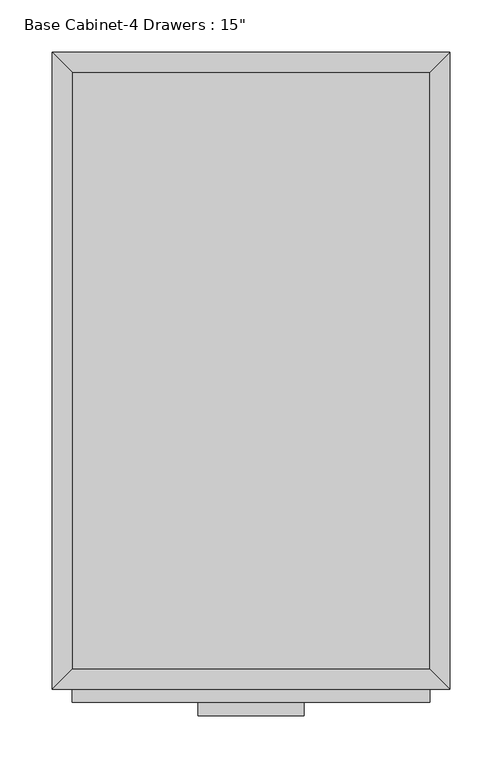
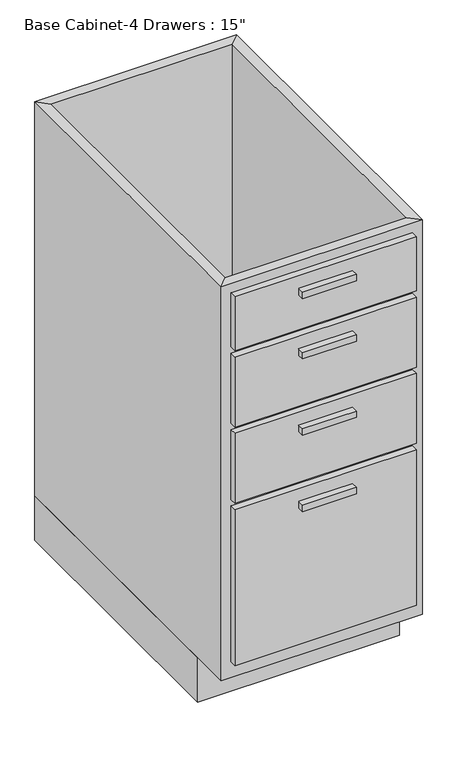
"""IFC4 building model written with IfcOpenShell, lengths in millimetres: furniture geometry."""

import ifcopenshell
import ifcopenshell.guid

model = None  # the IFC model being written
_history = None  # IfcOwnerHistory: only IFC2X3 demands one
_inside = {}  # id of a spatial element -> (the spatial element, [elements in it])
_under = {}  # id of a project, library or spatial element -> (it, [spatial elements below it])
_declared = {}  # id of a project -> (the project, [libraries it declares])
_typed = {}  # id of a type object -> (the type object, [elements of that type])
_made_of = {}  # id of a material, layer set ... -> (it, [elements and type objects made of it])


def new_model(schema):
    """Start an empty IFC model of exactly this schema.

    Asked for "IFC4X3", IfcOpenShell would pick the latest addendum, in which some entities
    have other attributes; the version numbers below select the first issue.
    IFC2X3 requires an IfcOwnerHistory on every rooted entity: one is made here for all.
    """
    global model, _history
    if schema == "IFC4X3":
        model = ifcopenshell.file(schema_version=(4, 3, 0, 0))
    else:
        model = ifcopenshell.file(schema=schema)
    _inside.clear()
    _under.clear()
    _declared.clear()
    _typed.clear()
    _made_of.clear()
    _history = None
    if model.schema == "IFC2X3":
        org = make("IfcOrganization", Name="unknown")
        user = make(
            "IfcPersonAndOrganization",
            ThePerson=make("IfcPerson", FamilyName="unknown"),
            TheOrganization=org,
        )
        app = make(
            "IfcApplication",
            ApplicationDeveloper=org,
            Version="unknown",
            ApplicationFullName="unknown",
            ApplicationIdentifier="unknown",
        )
        _history = make(
            "IfcOwnerHistory",
            OwningUser=user,
            OwningApplication=app,
            ChangeAction="ADDED",
            CreationDate=0,
        )
    return model


def make(cls, **values):
    """One entity of the class cls with the attributes given. An attribute that is None is left unset."""
    return model.create_entity(
        cls, **{name: value for name, value in values.items() if value is not None}
    )


def rooted(cls, **values):
    """An entity with a GlobalId (a new one), such as an element, a storey or a relation."""
    return make(cls, GlobalId=ifcopenshell.guid.new(), OwnerHistory=_history, **values)


def si_unit(unit_type, name, prefix=None):
    """IfcSIUnit, for example si_unit("LENGTHUNIT", "METRE", prefix="MILLI")."""
    return make("IfcSIUnit", UnitType=unit_type, Prefix=prefix, Name=name)


def assignment(units):
    """IfcUnitAssignment: the units of a project."""
    return None if units is None else make("IfcUnitAssignment", Units=units)


def point(xyz):
    """IfcCartesianPoint."""
    return None if xyz is None else make("IfcCartesianPoint", Coordinates=xyz)


def direction(xyz):
    """IfcDirection."""
    return None if xyz is None else make("IfcDirection", DirectionRatios=xyz)


def frame(location, z_axis=None, x_axis=None):
    """IfcAxis2Placement3D, a coordinate frame: its origin and axes. An axis left out is left unset."""
    return make(
        "IfcAxis2Placement3D",
        Location=point(location),
        Axis=direction(z_axis),
        RefDirection=direction(x_axis),
    )


def origin():
    """The frame at (0, 0, 0) with its axes left unset."""
    return frame((0.0, 0.0, 0.0))


def origin_with_axes():
    """The frame at (0, 0, 0) with the z axis (0, 0, 1) and the x axis (1, 0, 0) written out."""
    return frame((0.0, 0.0, 0.0), z_axis=(0.0, 0.0, 1.0), x_axis=(1.0, 0.0, 0.0))


def place(relative_to, where):
    """IfcLocalPlacement: puts the frame where relative to a parent placement (None: the world)."""
    return make(
        "IfcLocalPlacement", PlacementRelTo=relative_to, RelativePlacement=where
    )


def context(
    kind, dimensions, precision=None, world=None, true_north=None, identifier=None
):
    """IfcGeometricRepresentationContext, for example the 3D "Model" context."""
    return make(
        "IfcGeometricRepresentationContext",
        ContextIdentifier=identifier,
        ContextType=kind,
        CoordinateSpaceDimension=dimensions,
        Precision=precision,
        WorldCoordinateSystem=world,
        TrueNorth=true_north,
    )


def project(units=None, contexts=None):
    """IfcProject with its units and contexts."""
    return rooted(
        "IfcProject",
        Name="project",
        RepresentationContexts=contexts,
        UnitsInContext=assignment(units),
    )


def spatial(cls, under=None, at=None, **own):
    """A site, building, storey or space (cls), placed at a placement, below another one or the project."""
    s = rooted(cls, ObjectPlacement=at, **own)
    if under is not None:
        _under.setdefault(under.id(), (under, []))[1].append(s)
    return s


def polyline(points):
    """IfcPolyline through the points."""
    return make("IfcPolyline", Points=[point(p) for p in points])


def outline(outer, holes=None, kind="AREA"):
    """IfcArbitraryClosedProfileDef: a profile drawn as a closed curve; with holes, ...WithVoids."""
    if holes is None:
        return make("IfcArbitraryClosedProfileDef", ProfileType=kind, OuterCurve=outer)
    return make(
        "IfcArbitraryProfileDefWithVoids",
        ProfileType=kind,
        OuterCurve=outer,
        InnerCurves=holes,
    )


def extrude(swept, where, along, depth):
    """IfcExtrudedAreaSolid: the profile swept, set in the frame where, extruded along a direction by depth."""
    return make(
        "IfcExtrudedAreaSolid",
        SweptArea=swept,
        Position=where,
        ExtrudedDirection=direction(along),
        Depth=depth,
    )


def faces_of(points, faces, orient=None, outer=None):
    """IfcFace entities. A face is a list of loops; a loop is a list of indices into points, from 0.

    orient and outer hold one flag for each loop. By default every Orientation is true, the
    first loop of a face is its IfcFaceOuterBound and the others are IfcFaceBound.
    """
    made = []
    for i, loops in enumerate(faces):
        bounds = []
        for j, loop in enumerate(loops):
            is_outer = j == 0 if outer is None else outer[i][j]
            bounds.append(
                make(
                    "IfcFaceOuterBound" if is_outer else "IfcFaceBound",
                    Bound=make("IfcPolyLoop", Polygon=[points[k] for k in loop]),
                    Orientation=True if orient is None else orient[i][j],
                )
            )
        made.append(make("IfcFace", Bounds=bounds))
    return made


def faceted_brep(points, faces, orient=None, outer=None, voids=None):
    """IfcFacetedBrep: a solid bounded by flat faces; with voids (closed shells), ...WithVoids."""
    shared = [point(p) for p in points]
    hull = make("IfcClosedShell", CfsFaces=faces_of(shared, faces, orient, outer))
    if voids is None:
        return make("IfcFacetedBrep", Outer=hull)
    return make(
        "IfcFacetedBrepWithVoids",
        Outer=hull,
        Voids=[
            make(cls, CfsFaces=faces_of(shared, fs, o, b)) for cls, fs, o, b in voids
        ],
    )


def shape(context_of_items, identifier, shape_type, items):
    """IfcShapeRepresentation: the items that make up one representation, for example the "Body"."""
    return make(
        "IfcShapeRepresentation",
        ContextOfItems=context_of_items,
        RepresentationIdentifier=identifier,
        RepresentationType=shape_type,
        Items=items,
    )


def source(mapping_origin, context_of_items, identifier, shape_type, items):
    """IfcRepresentationMap: a shape defined once, which mapped items show again and again."""
    return make(
        "IfcRepresentationMap",
        MappingOrigin=mapping_origin,
        MappedRepresentation=shape(context_of_items, identifier, shape_type, items),
    )


def transform(
    local_origin,
    x_axis=None,
    y_axis=None,
    z_axis=None,
    scale=None,
    scale2=None,
    scale3=None,
    uniform=True,
):
    """IfcCartesianTransformationOperator3D, or its non-uniform kind. x_axis, y_axis, z_axis: its Axis1, 2, 3."""
    if uniform:
        return make(
            "IfcCartesianTransformationOperator3D",
            Axis1=direction(x_axis),
            Axis2=direction(y_axis),
            LocalOrigin=point(local_origin),
            Scale=scale,
            Axis3=direction(z_axis),
        )
    return make(
        "IfcCartesianTransformationOperator3DnonUniform",
        Axis1=direction(x_axis),
        Axis2=direction(y_axis),
        LocalOrigin=point(local_origin),
        Scale=scale,
        Axis3=direction(z_axis),
        Scale2=scale2,
        Scale3=scale3,
    )


def mapped(mapping_source, mapping_target):
    """IfcMappedItem: shows the shape of a source again, moved by a transform."""
    return make(
        "IfcMappedItem", MappingSource=mapping_source, MappingTarget=mapping_target
    )


def made_of(thing, what):
    """Note that an element or type object is made of a material, layer set ...; save() writes the relation."""
    if what is not None:
        _made_of.setdefault(what.id(), (what, []))[1].append(thing)
    return thing


def element(
    cls,
    number,
    at=None,
    inside=None,
    cuts=None,
    type_object=None,
    material=None,
    context=None,
    identifier="Body",
    shape_type=None,
    held_by="IfcProductDefinitionShape",
    body=None,
    shapes=None,
    **own,
):
    """One element of the class cls, such as IfcWall. Its Tag is "e" and its number.

    at: its placement. inside: the storey or other place that contains it. cuts: it is an
    opening in that element (IfcRelVoidsElement). A single representation is given by context,
    identifier, shape_type and body (its items); several are given by shapes. held_by: the class
    of the entity that holds the representations. save() writes the other relations.
    """
    e = rooted(cls, Tag="e%d" % number, ObjectPlacement=at, **own)
    if body is not None:
        shapes = [shape(context, identifier, shape_type, body)]
    if shapes is not None:
        e.Representation = make(held_by, Representations=shapes)
    if inside is not None:
        _inside.setdefault(inside.id(), (inside, []))[1].append(e)
    if cuts is not None:
        rooted(
            "IfcRelVoidsElement", RelatingBuildingElement=cuts, RelatedOpeningElement=e
        )
    if type_object is not None:
        _typed.setdefault(type_object.id(), (type_object, []))[1].append(e)
    return made_of(e, material)


def aggregate(whole, parts):
    """IfcRelAggregates: a whole, such as a stair, and the parts it consists of."""
    return rooted("IfcRelAggregates", RelatingObject=whole, RelatedObjects=parts)


def save(model, path):
    """Write the relations noted so far, then the file.

    IfcRelAggregates (storeys below a building ...), IfcRelContainedInSpatialStructure (elements
    in a storey), IfcRelDefinesByType, IfcRelAssociatesMaterial and IfcRelDeclares: one each for
    every whole, place, type object, material and project.
    """
    for whole, parts in _under.values():
        aggregate(whole, parts)
    for where, things in _inside.values():
        rooted(
            "IfcRelContainedInSpatialStructure",
            RelatedElements=things,
            RelatingStructure=where,
        )
    for kind, things in _typed.values():
        rooted("IfcRelDefinesByType", RelatedObjects=things, RelatingType=kind)
    for what, things in _made_of.values():
        rooted("IfcRelAssociatesMaterial", RelatedObjects=things, RelatingMaterial=what)
    for by, libraries in _declared.values():
        rooted("IfcRelDeclares", RelatingContext=by, RelatedDefinitions=libraries)
    model.write(path)


def furniture_a33faecb(model_context):
    return source(origin(), model_context, "Body", "SolidModel", [
        extrude(outline(polyline([(69.5377049, -635.0), (-32.0622951, -635.0), (-32.0622951, -622.3), (69.5377049, -622.3), (69.5377049, -635.0)])), frame((0.0, 0.0, 819.15), z_axis=(0.0, 0.0, 1.0), x_axis=(1.0, 0.0, 0.0)), (0.0, 0.0, 1.0), 12.7),
        extrude(outline(polyline([(69.5377049, -635.0), (-32.0622951, -635.0), (-32.0622951, -622.3), (69.5377049, -622.3), (69.5377049, -635.0)])), frame((0.0, 0.0, 698.5), z_axis=(0.0, 0.0, 1.0), x_axis=(1.0, 0.0, 0.0)), (0.0, 0.0, 1.0), 12.7),
        extrude(outline(polyline([(69.5377049, -635.0), (-32.0622951, -635.0), (-32.0622951, -622.3), (69.5377049, -622.3), (69.5377049, -635.0)])), frame((0.0, 0.0, 546.1), z_axis=(0.0, 0.0, 1.0), x_axis=(1.0, 0.0, 0.0)), (0.0, 0.0, 1.0), 12.7),
        extrude(outline(polyline([(69.5377049, -635.0), (-32.0622951, -635.0), (-32.0622951, -622.3), (69.5377049, -622.3), (69.5377049, -635.0)])), frame((0.0, 0.0, 393.7), z_axis=(0.0, 0.0, 1.0), x_axis=(1.0, 0.0, 0.0)), (0.0, 0.0, 1.0), 12.7),
        extrude(outline(polyline([(190.1877049, -622.3), (-152.7122951, -622.3), (-152.7122951, -609.6), (190.1877049, -609.6), (190.1877049, -622.3)])), frame((0.0, 0.0, 749.3), z_axis=(0.0, 0.0, 1.0), x_axis=(1.0, 0.0, 0.0)), (0.0, 0.0, 1.0), 107.95),
        extrude(outline(polyline([(190.1877049, -622.3), (-152.7122951, -622.3), (-152.7122951, -609.6), (190.1877049, -609.6), (190.1877049, -622.3)])), frame((0.0, 0.0, 596.9), z_axis=(0.0, 0.0, 1.0), x_axis=(1.0, 0.0, 0.0)), (0.0, 0.0, 1.0), 139.7),
        extrude(outline(polyline([(190.1877049, -622.3), (-152.7122951, -622.3), (-152.7122951, -609.6), (190.1877049, -609.6), (190.1877049, -622.3)])), frame((0.0, 0.0, 444.5), z_axis=(0.0, 0.0, 1.0), x_axis=(1.0, 0.0, 0.0)), (0.0, 0.0, 1.0), 139.7),
        extrude(outline(polyline([(190.1877049, -622.3), (-152.7122951, -622.3), (-152.7122951, -609.6), (190.1877049, -609.6), (190.1877049, -622.3)])), frame((0.0, 0.0, 120.65), z_axis=(0.0, 0.0, 1.0), x_axis=(1.0, 0.0, 0.0)), (0.0, 0.0, 1.0), 311.15),
        extrude(outline(polyline([(190.1877049, -19.05), (190.1877049, -590.55), (-152.7122951, -590.55), (-152.7122951, -19.05), (190.1877049, -19.05)])), frame((0.0, 0.0, 88.9), z_axis=(0.0, 0.0, 1.0), x_axis=(1.0, 0.0, 0.0)), (0.0, 0.0, 1.0), 19.05),
        faceted_brep([(190.1877049, -590.55, 876.3), (190.1877049, -590.55, 88.9), (-152.7122951, -590.55, 88.9), (-152.7122951, -590.55, 876.3), (209.2377049, -609.6, 876.3), (-171.7622951, -609.6, 876.3), (209.2377049, -609.6, 88.9), (-171.7622951, -609.6, 88.9), (-152.7122951, -19.05, 88.9), (-152.7122951, -19.05, 876.3), (-171.7622951, 0.0, 876.3), (-171.7622951, 0.0, 88.9), (190.1877049, -19.05, 88.9), (190.1877049, -19.05, 876.3), (209.2377049, 0.0, 876.3), (209.2377049, 0.0, 88.9)], [[[0, 1, 2, 3]], [[4, 0, 3, 5]], [[6, 4, 5, 7]], [[1, 6, 7, 2]], [[3, 2, 8, 9]], [[5, 3, 9, 10]], [[7, 5, 10, 11]], [[2, 7, 11, 8]], [[9, 8, 12, 13]], [[10, 9, 13, 14]], [[11, 10, 14, 15]], [[8, 11, 15, 12]], [[13, 12, 1, 0]], [[14, 13, 0, 4]], [[15, 14, 4, 6]], [[12, 15, 6, 1]]]),
        extrude(outline(polyline([(209.2377049, 0.0), (209.2377049, -533.4), (-171.7622951, -533.4), (-171.7622951, 0.0), (209.2377049, 0.0)])), origin_with_axes(), (0.0, 0.0, 1.0), 88.9),
    ])


if __name__ == "__main__":
    model = new_model("IFC4")
    model_context = context("Model", 3, world=origin())
    ifc_project = project(units=[si_unit("LENGTHUNIT", "METRE", prefix="MILLI")], contexts=[model_context])
    site = spatial("IfcSite", under=ifc_project)
    building = spatial("IfcBuilding", under=site)
    placement = place(None, origin())
    furniture_shape = furniture_a33faecb(model_context)
    element("IfcFurniture", 1, ObjectType="Base Cabinet-4 Drawers : 15\"", at=placement, inside=building, context=model_context, shape_type="MappedRepresentation", body=[
        mapped(furniture_shape, transform((0.0, 0.0, 0.0), x_axis=(1.0, 0.0, 0.0), y_axis=(0.0, 1.0, 0.0), z_axis=(0.0, 0.0, 1.0))),
    ])
    save(model, "model.ifc")

# Revit data of these elements
# Type "Base Cabinet-4 Drawers : 15\""
#   Assembly Code = "C1030410"
#   Depth = 2' - 0"
#   Height = 2' - 10 1/2"
#   Toe Depth = 0' - 3"
#   Toe Height = 0' - 3 1/2"
#   Width = 1' - 3"
#   Cabinet Material = none
#   Door/Drawer Material = none
#   Handle Material = Cabinets - Handles
#   Default Elevation = 0
# Element 1 (IfcFurniture, "Base Cabinet-4 Drawers : 15\"")
#   Materials on its faces: "Cabinets", "Cabinets - Handles"
# Materials
#   "Cabinets - Handles": class "Metal", colour RGB 57 57 57, transparency 0
#   "Cabinets": class "Miscellaneous", colour RGB 249 249 249, transparency 0
